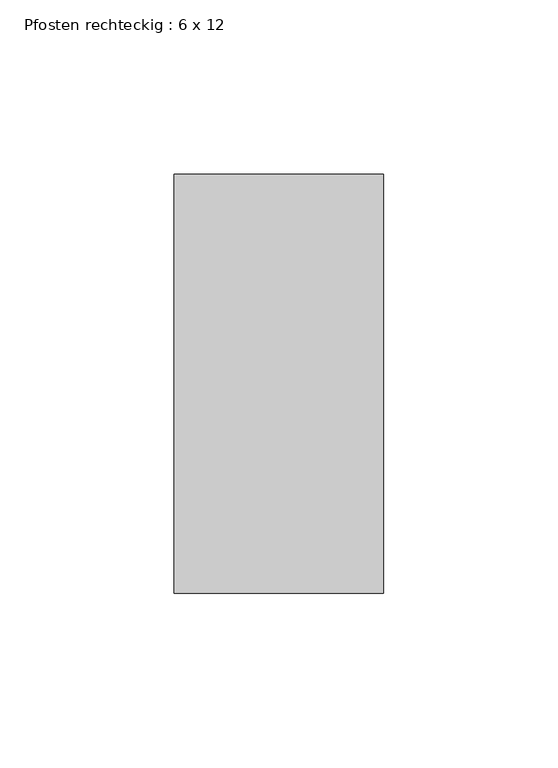
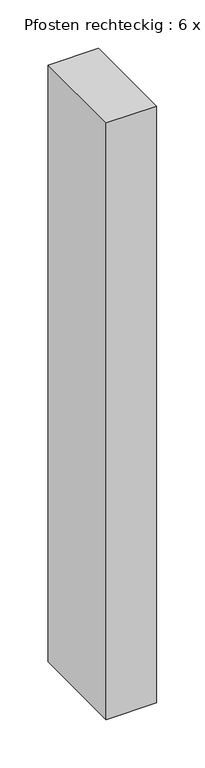
"""IFC4 building model written with IfcOpenShell, lengths in millimetres: member geometry, Pfosten rechteckig : 6 x 12."""

from ifc_helpers import new_model, si_unit, frame, origin, place, context, project, spatial, polyline, outline, extrude, source, transform, mapped, element, save


def pfosten_rechteckig_6_x_12_6e5f5406(model_context):
    return source(origin(), model_context, "Body", "SweptSolid", [
        extrude(outline(polyline([(0.0, 60.0), (0.0, -60.0), (-60.0, -60.0), (-60.0, 60.0), (0.0, 60.0)])), frame((0.0, 0.0, -752.9462629), z_axis=(0.0, 0.0, 1.0), x_axis=(1.0, 0.0, 0.0)), (0.0, 0.0, 1.0), 752.9462629),
    ])


if __name__ == "__main__":
    model = new_model("IFC4")
    model_context = context("Model", 3, world=origin())
    ifc_project = project(units=[si_unit("LENGTHUNIT", "METRE", prefix="MILLI")], contexts=[model_context])
    site = spatial("IfcSite", under=ifc_project)
    building = spatial("IfcBuilding", under=site)
    placement = place(None, origin())
    pfosten_rechteckig_6_x_12_shape = pfosten_rechteckig_6_x_12_6e5f5406(model_context)
    element("IfcMember", 1, ObjectType="Pfosten rechteckig : 6 x 12", at=placement, inside=building, context=model_context, shape_type="MappedRepresentation", body=[
        mapped(pfosten_rechteckig_6_x_12_shape, transform((0.0, 0.0, 0.0), x_axis=(1.0, 0.0, 0.0), y_axis=(0.0, 1.0, 0.0), z_axis=(0.0, 0.0, 1.0))),
    ])
    save(model, "model.ifc")

# Revit data of these elements
# Type "Pfosten rechteckig : 6 x 12"
#   built-in parameter 1007304 = 0.393701 (stored number, unit not read)
#   built-in parameter 1007301 = 0.0984252 (stored number, unit not read)
#   built-in parameter 1007300 = 0.0984252 (stored number, unit not read)
# Element 1 (IfcMember, "Pfosten rechteckig : 6 x 12")
#   Materials on its faces: "Metall - verzinkt"
# Materials
#   "Metall - verzinkt": class "Allgemeines", colour RGB 200 200 200, transparency 0, Cost = 0
